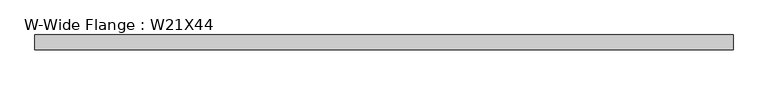
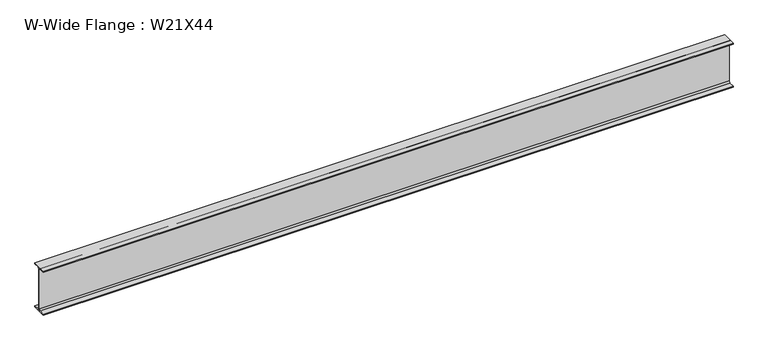
"""IFC4 building model written with IfcOpenShell, lengths in millimetres: beam geometry, W-Wide Flange : W21X44."""

from ifc_helpers import new_model, si_unit, point, frame, frame_2d, origin, place, context, project, spatial, polyline, circle_curve, trimmed, segment, composite_curve, outline, extrude, source, transform, mapped, element, save


def w_wide_flange_w21x44_b21c43a2(model_context):
    return source(origin(), model_context, "Body", "SweptSolid", [
        extrude(outline(composite_curve([segment(polyline([(82.55, -251.46), (82.55, -262.89), (-82.55, -262.89), (-82.55, -251.46), (-21.59, -251.46)]), True, "CONTINUOUS"), segment(trimmed(circle_curve(frame_2d((-21.59, -234.315)), 17.145), [point((-21.59, -251.46))], [point((-4.445, -234.315))], True, "CARTESIAN"), True, "CONTINUOUS"), segment(polyline([(-4.445, -234.315), (-4.445, 234.315)]), True, "CONTINUOUS"), segment(trimmed(circle_curve(frame_2d((-21.59, 234.315)), 17.145), [point((-4.445, 234.315))], [point((-21.59, 251.46))], True, "CARTESIAN"), True, "CONTINUOUS"), segment(polyline([(-21.59, 251.46), (-82.55, 251.46), (-82.55, 262.89), (82.55, 262.89), (82.55, 251.46), (21.59, 251.46)]), True, "CONTINUOUS"), segment(trimmed(circle_curve(frame_2d((21.59, 234.315)), 17.145), [point((21.59, 251.46))], [point((4.445, 234.315))], True, "CARTESIAN"), True, "CONTINUOUS"), segment(polyline([(4.445, 234.315), (4.445, -234.315)]), True, "CONTINUOUS"), segment(trimmed(circle_curve(frame_2d((21.59, -234.315)), 17.145), [point((4.445, -234.315))], [point((21.59, -251.46))], True, "CARTESIAN"), True, "CONTINUOUS"), segment(polyline([(21.59, -251.46), (82.55, -251.46)]), True, "CONTINUOUS")], self_intersect=False)), frame((-3911.6, 0.0, 0.0), z_axis=(1.0, 0.0, 0.0), x_axis=(0.0, 1.0, 0.0)), (0.0, 0.0, 1.0), 7823.2),
    ])


if __name__ == "__main__":
    model = new_model("IFC4")
    model_context = context("Model", 3, world=origin())
    ifc_project = project(units=[si_unit("LENGTHUNIT", "METRE", prefix="MILLI")], contexts=[model_context])
    site = spatial("IfcSite", under=ifc_project)
    building = spatial("IfcBuilding", under=site)
    placement = place(None, origin())
    w_wide_flange_w21x44_shape = w_wide_flange_w21x44_b21c43a2(model_context)
    element("IfcBeam", 1, ObjectType="W-Wide Flange : W21X44", at=placement, inside=building, context=model_context, shape_type="MappedRepresentation", body=[
        mapped(w_wide_flange_w21x44_shape, transform((0.0, 0.0, 0.0), x_axis=(1.0, 0.0, 0.0), y_axis=(0.0, 1.0, 0.0), z_axis=(0.0, 0.0, 1.0))),
    ])
    save(model, "model.ifc")

# Revit data of these elements
# Type "W-Wide Flange : W21X44"
#   Assembly Code = "B10"
#   W = 44
#   Length [instance default] = 5' - 0"
#   bf = 0' - 6 1/2"
#   d = 1' - 8.7"
#   k = 0' - 1 1/8"
#   k2 = 0' - 0.675"
#   tf = 0' - 0.45"
#   tw = 0' - 0.35"
#   A = 0.0902778 SF
#   Structural Material [instance default] = Steel ASTM A992
# Element 1 (IfcBeam, "W-Wide Flange : W21X44")
#   Materials on its faces: "Steel ASTM A992"
# Materials
#   "Steel ASTM A992": class "Metal", colour RGB 199 199 199, transparency 0, Description = "Structural steel 50ksi", Cost = 0
